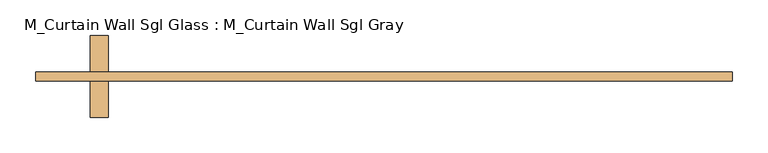
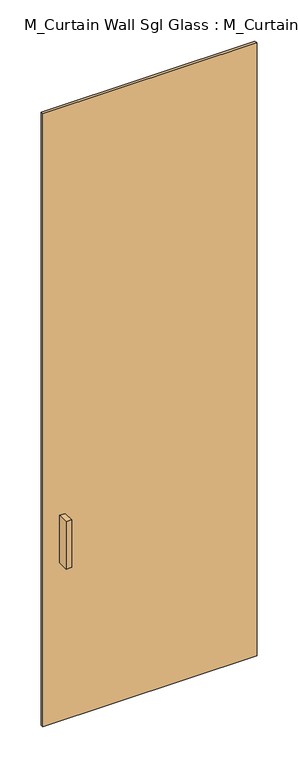
"""IFC4 building model written with IfcOpenShell, lengths in millimetres: door geometry, M_Curtain Wall Sgl Glass : M_Curtain Wall Sgl Gray."""

import ifcopenshell
import ifcopenshell.guid

model = None  # the IFC model being written
_history = None  # IfcOwnerHistory: only IFC2X3 demands one
_inside = {}  # id of a spatial element -> (the spatial element, [elements in it])
_under = {}  # id of a project, library or spatial element -> (it, [spatial elements below it])
_declared = {}  # id of a project -> (the project, [libraries it declares])
_typed = {}  # id of a type object -> (the type object, [elements of that type])
_made_of = {}  # id of a material, layer set ... -> (it, [elements and type objects made of it])


def new_model(schema):
    """Start an empty IFC model of exactly this schema.

    Asked for "IFC4X3", IfcOpenShell would pick the latest addendum, in which some entities
    have other attributes; the version numbers below select the first issue.
    IFC2X3 requires an IfcOwnerHistory on every rooted entity: one is made here for all.
    """
    global model, _history
    if schema == "IFC4X3":
        model = ifcopenshell.file(schema_version=(4, 3, 0, 0))
    else:
        model = ifcopenshell.file(schema=schema)
    _inside.clear()
    _under.clear()
    _declared.clear()
    _typed.clear()
    _made_of.clear()
    _history = None
    if model.schema == "IFC2X3":
        org = make("IfcOrganization", Name="unknown")
        user = make(
            "IfcPersonAndOrganization",
            ThePerson=make("IfcPerson", FamilyName="unknown"),
            TheOrganization=org,
        )
        app = make(
            "IfcApplication",
            ApplicationDeveloper=org,
            Version="unknown",
            ApplicationFullName="unknown",
            ApplicationIdentifier="unknown",
        )
        _history = make(
            "IfcOwnerHistory",
            OwningUser=user,
            OwningApplication=app,
            ChangeAction="ADDED",
            CreationDate=0,
        )
    return model


def make(cls, **values):
    """One entity of the class cls with the attributes given. An attribute that is None is left unset."""
    return model.create_entity(
        cls, **{name: value for name, value in values.items() if value is not None}
    )


def rooted(cls, **values):
    """An entity with a GlobalId (a new one), such as an element, a storey or a relation."""
    return make(cls, GlobalId=ifcopenshell.guid.new(), OwnerHistory=_history, **values)


def si_unit(unit_type, name, prefix=None):
    """IfcSIUnit, for example si_unit("LENGTHUNIT", "METRE", prefix="MILLI")."""
    return make("IfcSIUnit", UnitType=unit_type, Prefix=prefix, Name=name)


def assignment(units):
    """IfcUnitAssignment: the units of a project."""
    return None if units is None else make("IfcUnitAssignment", Units=units)


def point(xyz):
    """IfcCartesianPoint."""
    return None if xyz is None else make("IfcCartesianPoint", Coordinates=xyz)


def direction(xyz):
    """IfcDirection."""
    return None if xyz is None else make("IfcDirection", DirectionRatios=xyz)


def frame(location, z_axis=None, x_axis=None):
    """IfcAxis2Placement3D, a coordinate frame: its origin and axes. An axis left out is left unset."""
    return make(
        "IfcAxis2Placement3D",
        Location=point(location),
        Axis=direction(z_axis),
        RefDirection=direction(x_axis),
    )


def origin():
    """The frame at (0, 0, 0) with its axes left unset."""
    return frame((0.0, 0.0, 0.0))


def origin_with_axes():
    """The frame at (0, 0, 0) with the z axis (0, 0, 1) and the x axis (1, 0, 0) written out."""
    return frame((0.0, 0.0, 0.0), z_axis=(0.0, 0.0, 1.0), x_axis=(1.0, 0.0, 0.0))


def place(relative_to, where):
    """IfcLocalPlacement: puts the frame where relative to a parent placement (None: the world)."""
    return make(
        "IfcLocalPlacement", PlacementRelTo=relative_to, RelativePlacement=where
    )


def context(
    kind, dimensions, precision=None, world=None, true_north=None, identifier=None
):
    """IfcGeometricRepresentationContext, for example the 3D "Model" context."""
    return make(
        "IfcGeometricRepresentationContext",
        ContextIdentifier=identifier,
        ContextType=kind,
        CoordinateSpaceDimension=dimensions,
        Precision=precision,
        WorldCoordinateSystem=world,
        TrueNorth=true_north,
    )


def project(units=None, contexts=None):
    """IfcProject with its units and contexts."""
    return rooted(
        "IfcProject",
        Name="project",
        RepresentationContexts=contexts,
        UnitsInContext=assignment(units),
    )


def spatial(cls, under=None, at=None, **own):
    """A site, building, storey or space (cls), placed at a placement, below another one or the project."""
    s = rooted(cls, ObjectPlacement=at, **own)
    if under is not None:
        _under.setdefault(under.id(), (under, []))[1].append(s)
    return s


def polyline(points):
    """IfcPolyline through the points."""
    return make("IfcPolyline", Points=[point(p) for p in points])


def outline(outer, holes=None, kind="AREA"):
    """IfcArbitraryClosedProfileDef: a profile drawn as a closed curve; with holes, ...WithVoids."""
    if holes is None:
        return make("IfcArbitraryClosedProfileDef", ProfileType=kind, OuterCurve=outer)
    return make(
        "IfcArbitraryProfileDefWithVoids",
        ProfileType=kind,
        OuterCurve=outer,
        InnerCurves=holes,
    )


def extrude(swept, where, along, depth):
    """IfcExtrudedAreaSolid: the profile swept, set in the frame where, extruded along a direction by depth."""
    return make(
        "IfcExtrudedAreaSolid",
        SweptArea=swept,
        Position=where,
        ExtrudedDirection=direction(along),
        Depth=depth,
    )


def shape(context_of_items, identifier, shape_type, items):
    """IfcShapeRepresentation: the items that make up one representation, for example the "Body"."""
    return make(
        "IfcShapeRepresentation",
        ContextOfItems=context_of_items,
        RepresentationIdentifier=identifier,
        RepresentationType=shape_type,
        Items=items,
    )


def source(mapping_origin, context_of_items, identifier, shape_type, items):
    """IfcRepresentationMap: a shape defined once, which mapped items show again and again."""
    return make(
        "IfcRepresentationMap",
        MappingOrigin=mapping_origin,
        MappedRepresentation=shape(context_of_items, identifier, shape_type, items),
    )


def transform(
    local_origin,
    x_axis=None,
    y_axis=None,
    z_axis=None,
    scale=None,
    scale2=None,
    scale3=None,
    uniform=True,
):
    """IfcCartesianTransformationOperator3D, or its non-uniform kind. x_axis, y_axis, z_axis: its Axis1, 2, 3."""
    if uniform:
        return make(
            "IfcCartesianTransformationOperator3D",
            Axis1=direction(x_axis),
            Axis2=direction(y_axis),
            LocalOrigin=point(local_origin),
            Scale=scale,
            Axis3=direction(z_axis),
        )
    return make(
        "IfcCartesianTransformationOperator3DnonUniform",
        Axis1=direction(x_axis),
        Axis2=direction(y_axis),
        LocalOrigin=point(local_origin),
        Scale=scale,
        Axis3=direction(z_axis),
        Scale2=scale2,
        Scale3=scale3,
    )


def mapped(mapping_source, mapping_target):
    """IfcMappedItem: shows the shape of a source again, moved by a transform."""
    return make(
        "IfcMappedItem", MappingSource=mapping_source, MappingTarget=mapping_target
    )


def made_of(thing, what):
    """Note that an element or type object is made of a material, layer set ...; save() writes the relation."""
    if what is not None:
        _made_of.setdefault(what.id(), (what, []))[1].append(thing)
    return thing


def element(
    cls,
    number,
    at=None,
    inside=None,
    cuts=None,
    type_object=None,
    material=None,
    context=None,
    identifier="Body",
    shape_type=None,
    held_by="IfcProductDefinitionShape",
    body=None,
    shapes=None,
    **own,
):
    """One element of the class cls, such as IfcWall. Its Tag is "e" and its number.

    at: its placement. inside: the storey or other place that contains it. cuts: it is an
    opening in that element (IfcRelVoidsElement). A single representation is given by context,
    identifier, shape_type and body (its items); several are given by shapes. held_by: the class
    of the entity that holds the representations. save() writes the other relations.
    """
    e = rooted(cls, Tag="e%d" % number, ObjectPlacement=at, **own)
    if body is not None:
        shapes = [shape(context, identifier, shape_type, body)]
    if shapes is not None:
        e.Representation = make(held_by, Representations=shapes)
    if inside is not None:
        _inside.setdefault(inside.id(), (inside, []))[1].append(e)
    if cuts is not None:
        rooted(
            "IfcRelVoidsElement", RelatingBuildingElement=cuts, RelatedOpeningElement=e
        )
    if type_object is not None:
        _typed.setdefault(type_object.id(), (type_object, []))[1].append(e)
    return made_of(e, material)


def aggregate(whole, parts):
    """IfcRelAggregates: a whole, such as a stair, and the parts it consists of."""
    return rooted("IfcRelAggregates", RelatingObject=whole, RelatedObjects=parts)


def save(model, path):
    """Write the relations noted so far, then the file.

    IfcRelAggregates (storeys below a building ...), IfcRelContainedInSpatialStructure (elements
    in a storey), IfcRelDefinesByType, IfcRelAssociatesMaterial and IfcRelDeclares: one each for
    every whole, place, type object, material and project.
    """
    for whole, parts in _under.values():
        aggregate(whole, parts)
    for where, things in _inside.values():
        rooted(
            "IfcRelContainedInSpatialStructure",
            RelatedElements=things,
            RelatingStructure=where,
        )
    for kind, things in _typed.values():
        rooted("IfcRelDefinesByType", RelatedObjects=things, RelatingType=kind)
    for what, things in _made_of.values():
        rooted("IfcRelAssociatesMaterial", RelatedObjects=things, RelatingMaterial=what)
    for by, libraries in _declared.values():
        rooted("IfcRelDeclares", RelatingContext=by, RelatedDefinitions=libraries)
    model.write(path)


def m_curtain_wall_sgl_glass_m_curtain_wall_sgl_gray_3072e32e(model_context):
    return source(origin(), model_context, "Body", "SweptSolid", [
        extrude(outline(polyline([(-385.9, 12.5), (-385.9, -38.3), (-411.3, -38.3), (-411.3, 12.5), (-385.9, 12.5)])), frame((0.0, 0.0, 762.0), z_axis=(0.0, 0.0, 1.0), x_axis=(1.0, 0.0, 0.0)), (0.0, 0.0, 1.0), 228.6),
        extrude(outline(polyline([(-411.3, -101.8), (-411.3, -51.0), (-385.9, -51.0), (-385.9, -101.8), (-411.3, -101.8)])), frame((0.0, 0.0, 762.0), z_axis=(0.0, 0.0, 1.0), x_axis=(1.0, 0.0, 0.0)), (0.0, 0.0, 1.0), 228.6),
        extrude(outline(polyline([(487.5, -51.0), (-487.5, -51.0), (-487.5, -38.3), (487.5, -38.3), (487.5, -51.0)])), origin_with_axes(), (0.0, 0.0, 1.0), 2950.0),
    ])


if __name__ == "__main__":
    model = new_model("IFC4")
    model_context = context("Model", 3, world=origin())
    ifc_project = project(units=[si_unit("LENGTHUNIT", "METRE", prefix="MILLI")], contexts=[model_context])
    site = spatial("IfcSite", under=ifc_project)
    building = spatial("IfcBuilding", under=site)
    placement = place(None, origin())
    m_curtain_wall_sgl_glass_m_curtain_wall_sgl_gray_shape = m_curtain_wall_sgl_glass_m_curtain_wall_sgl_gray_3072e32e(model_context)
    element("IfcDoor", 1, ObjectType="M_Curtain Wall Sgl Glass : M_Curtain Wall Sgl Gray", at=placement, inside=building, context=model_context, shape_type="MappedRepresentation", body=[
        mapped(m_curtain_wall_sgl_glass_m_curtain_wall_sgl_gray_shape, transform((0.0, 0.0, 0.0), x_axis=(1.0, 0.0, 0.0), y_axis=(0.0, 1.0, 0.0), z_axis=(0.0, 0.0, 1.0))),
    ])
    save(model, "model.ifc")

# Revit data of these elements
# Type "M_Curtain Wall Sgl Glass : M_Curtain Wall Sgl Gray"
#   Model = "12345667"
#   Manufacturer = "Dublin Doors"
#   Description = "Single Flush door"
#   Type Mark = "48"
#   COBie.Type.CreatedBy = "design@eagle.com"
#   COBie.Type.CreatedOn = "2016-09-13T05:47:35"
#   COBie.Type.Name = "Doors_M_Curtain Wall Sgl Glass_M_Curtain Wall Sgl Gray"
#   COBie.Type.Category = "23-30 10 00 : Doors"
#   COBie.Type.Description = "Single Flush door"
#   COBie.Type.Manufacturer = "Dublin Doors"
#   COBie.Type.ModelNumber = "12345667"
#   Construction Type Id = "opn-d36"
#   Analytic Construction = "Wood panel"
#   COBie.Type.ReplacementCost = 0
#   Offset = 51 mm
#   Heat Transfer Coefficient (U) = 3.8042 W/(m²·K)
#   COBie.Type = yes
#   Function = 1
#   Glazing Material = Door - Frame(1)
#   Visual Light Transmittance = 0
#   Solar Heat Gain Coefficient = 0
# Element 1 (IfcDoor, "M_Curtain Wall Sgl Glass : M_Curtain Wall Sgl Gray")
#   Materials on its faces: "Aluminum", "Door - Frame(1)"
# Materials
#   "Door - Frame(1)": class "Miscellaneous", colour RGB 128 128 128, transparency 0, Cost = 0
#   "Aluminum": class "Metal", colour RGB 247 247 247, transparency 0, Description = "Aluminum 6061", Cost = 0
